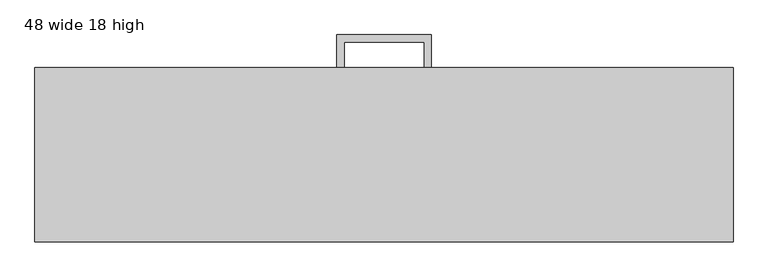
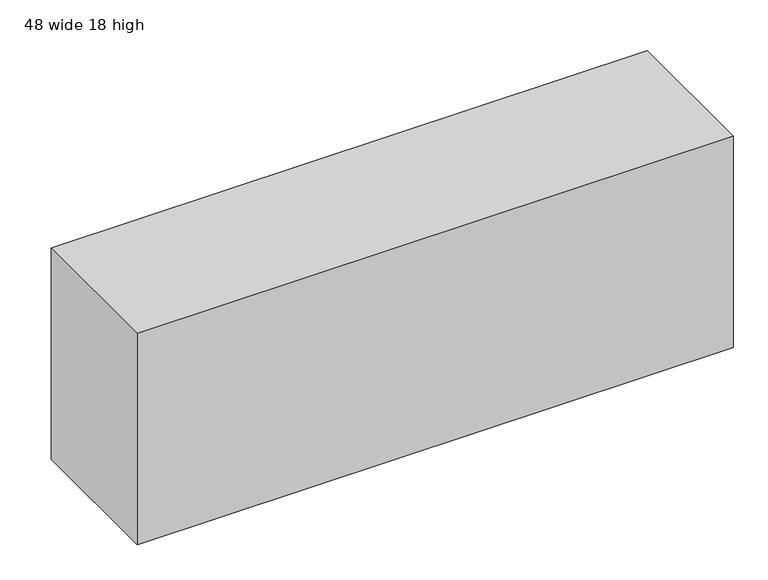
"""IFC4 building model written with IfcOpenShell, lengths in millimetres: furniture geometry, Binder Bin : 48 wide 18 high."""

from ifc_helpers import new_model, si_unit, frame, origin, place, context, project, spatial, polyline, outline, extrude, source, transform, mapped, element, save


def furniture_48_wide_18_high_2f3f987a(model_context):
    return source(origin(), model_context, "Body", "SweptSolid", [
        extrude(outline(polyline([(-69.85, 381.0), (-82.55, 381.0), (-82.55, 438.15), (82.55, 438.15), (82.55, 381.0), (69.85, 381.0), (69.85, 425.45), (-69.85, 425.45), (-69.85, 381.0)])), frame((0.0, 0.0, 1568.45), z_axis=(0.0, 0.0, 1.0), x_axis=(1.0, 0.0, 0.0)), (0.0, 0.0, 1.0), 12.7),
        extrude(outline(polyline([(609.6, 76.2), (-609.6, 76.2), (-609.6, 381.0), (609.6, 381.0), (609.6, 76.2)])), frame((0.0, 0.0, 1524.0), z_axis=(0.0, 0.0, 1.0), x_axis=(1.0, 0.0, 0.0)), (0.0, 0.0, 1.0), 457.2),
    ])


if __name__ == "__main__":
    model = new_model("IFC4")
    model_context = context("Model", 3, world=origin())
    ifc_project = project(units=[si_unit("LENGTHUNIT", "METRE", prefix="MILLI")], contexts=[model_context])
    site = spatial("IfcSite", under=ifc_project)
    building = spatial("IfcBuilding", under=site)
    placement = place(None, origin())
    furniture_48_wide_18_high_shape = furniture_48_wide_18_high_2f3f987a(model_context)
    element("IfcFurniture", 1, ObjectType="Binder Bin : 48 wide 18 high", at=placement, inside=building, context=model_context, shape_type="MappedRepresentation", body=[
        mapped(furniture_48_wide_18_high_shape, transform((0.0, 0.0, 0.0), x_axis=(1.0, 0.0, 0.0), y_axis=(0.0, 1.0, 0.0), z_axis=(0.0, 0.0, 1.0))),
    ])
    save(model, "model.ifc")

# Revit data of these elements
# Type "Binder Bin : 48 wide 18 high"
#   Model = "BIN-4818"
#   Manufacturer = "Corporate Concepts"
#   Type Mark = "BN-2"
#   Model = "BIN-4818"
#   Manufacturer = "Corporate Concepts"
#   Cost = 675
#   Width = 4' - 0"
#   Mounting Height [instance default] = 4' - 6"
#   Height = 1' - 6"
#   Cost = 675
#   Type Image = Binder Bin.png
#   Default Elevation = 0
# Element 1 (IfcFurniture, "Binder Bin : 48 wide 18 high")
#   Mounting Height = 5' - 0"
